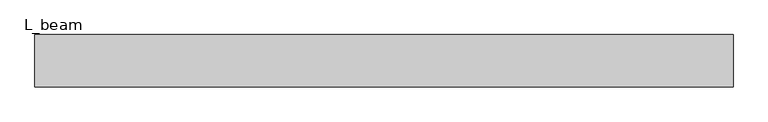
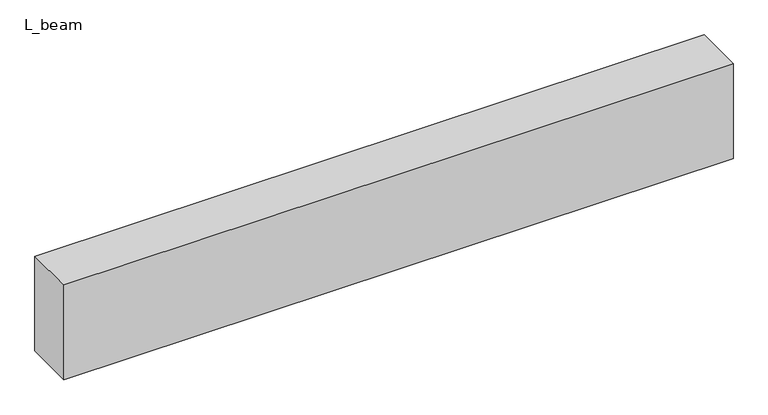
"""IFC4 building model written with IfcOpenShell, lengths in millimetres: beam geometry, 混凝土 - 矩形梁 : L_beam."""

from ifc_helpers import new_model, si_unit, frame, origin, place, context, project, spatial, polyline, outline, extrude, source, transform, mapped, element, save


def l_beam_a33c695f(model_context):
    return source(origin(), model_context, "Body", "SweptSolid", [
        extrude(outline(polyline([(2001.5, 150.0), (2001.5, -150.0), (-2001.5, -150.0), (-2001.5, 150.0), (2001.5, 150.0)])), frame((0.0, 0.0, -300.0), z_axis=(0.0, 0.0, 1.0), x_axis=(1.0, 0.0, 0.0)), (0.0, 0.0, 1.0), 600.0),
    ])


if __name__ == "__main__":
    model = new_model("IFC4")
    model_context = context("Model", 3, world=origin())
    ifc_project = project(units=[si_unit("LENGTHUNIT", "METRE", prefix="MILLI")], contexts=[model_context])
    site = spatial("IfcSite", under=ifc_project)
    building = spatial("IfcBuilding", under=site)
    placement = place(None, origin())
    l_beam_shape = l_beam_a33c695f(model_context)
    element("IfcBeam", 1, ObjectType="混凝土 - 矩形梁 : L_beam", at=placement, inside=building, context=model_context, shape_type="MappedRepresentation", body=[
        mapped(l_beam_shape, transform((0.0, 0.0, 0.0), x_axis=(1.0, 0.0, 0.0), y_axis=(0.0, 1.0, 0.0), z_axis=(0.0, 0.0, 1.0))),
    ])
    save(model, "model.ifc")

# Revit data of these elements
# Type "混凝土 - 矩形梁 : L_beam"
#   Length [instance default] = 1524 mm
#   b = 300 mm
#   h = 600 mm
#   Structural Material [instance default] = none
#   Assembly Code = ""
